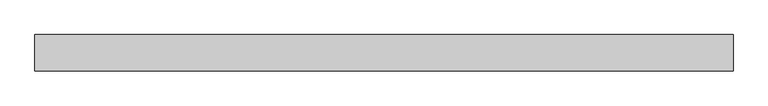
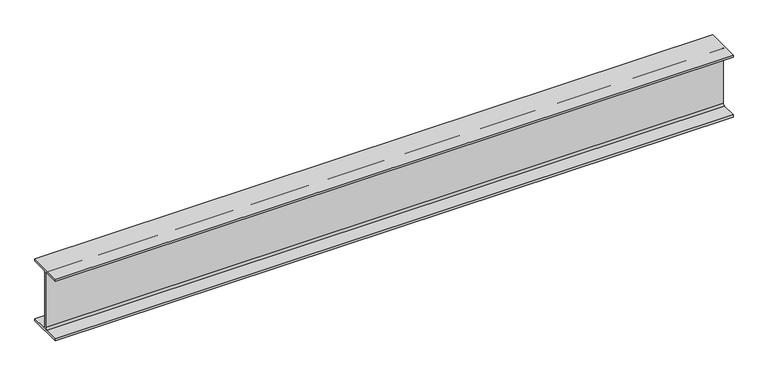
"""IFC4 building model written with IfcOpenShell, lengths in millimetres: beam geometry, Old_Steel Beam_H-KSD3502 : H_SB_ASB_H-250×125x6x9."""

from ifc_helpers import new_model, si_unit, point, frame, frame_2d, origin, place, context, project, spatial, polyline, circle_curve, trimmed, segment, composite_curve, outline, extrude, source, transform, mapped, element, save


def beam_c4c65e90(model_context):
    return source(origin(), model_context, "Body", "SweptSolid", [
        extrude(outline(composite_curve([segment(polyline([(82.5, -141.5), (82.5, -151.7), (-82.5, -151.7), (-82.5, -141.5), (-11.9, -141.5)]), True, "CONTINUOUS"), segment(trimmed(circle_curve(frame_2d((-11.9, -132.6)), 8.9), [point((-11.9, -141.5))], [point((-3.0, -132.6))], True, "CARTESIAN"), True, "CONTINUOUS"), segment(polyline([(-3.0, -132.6), (-3.0, 132.6)]), True, "CONTINUOUS"), segment(trimmed(circle_curve(frame_2d((-11.9, 132.6)), 8.9), [point((-3.0, 132.6))], [point((-11.9, 141.5))], True, "CARTESIAN"), True, "CONTINUOUS"), segment(polyline([(-11.9, 141.5), (-82.5, 141.5), (-82.5, 151.7), (82.5, 151.7), (82.5, 141.5), (11.9, 141.5)]), True, "CONTINUOUS"), segment(trimmed(circle_curve(frame_2d((11.9, 132.6)), 8.9), [point((11.9, 141.5))], [point((3.0, 132.6))], True, "CARTESIAN"), True, "CONTINUOUS"), segment(polyline([(3.0, 132.6), (3.0, -132.6)]), True, "CONTINUOUS"), segment(trimmed(circle_curve(frame_2d((11.9, -132.6)), 8.9), [point((3.0, -132.6))], [point((11.9, -141.5))], True, "CARTESIAN"), True, "CONTINUOUS"), segment(polyline([(11.9, -141.5), (82.5, -141.5)]), True, "CONTINUOUS")], self_intersect=False)), frame((-1494.5360727, 0.0, 0.0), z_axis=(1.0, 0.0, 0.0), x_axis=(0.0, 1.0, 0.0)), (0.0, 0.0, 1.0), 3149.3360727),
    ])


if __name__ == "__main__":
    model = new_model("IFC4")
    model_context = context("Model", 3, world=origin())
    ifc_project = project(units=[si_unit("LENGTHUNIT", "METRE", prefix="MILLI")], contexts=[model_context])
    site = spatial("IfcSite", under=ifc_project)
    building = spatial("IfcBuilding", under=site)
    placement = place(None, origin())
    beam_shape = beam_c4c65e90(model_context)
    element("IfcBeam", 1, ObjectType="Old_Steel Beam_H-KSD3502 : H_SB_ASB_H-250×125x6x9", at=placement, inside=building, context=model_context, shape_type="MappedRepresentation", body=[
        mapped(beam_shape, transform((0.0, 0.0, 0.0), x_axis=(1.0, 0.0, 0.0), y_axis=(0.0, 1.0, 0.0), z_axis=(0.0, 0.0, 1.0))),
    ])
    save(model, "model.ifc")

# Revit data of these elements
# Type "Old_Steel Beam_H-KSD3502 : H_SB_ASB_H-250×125x6x9"
#   Width = 12.5 cm
#   Web Thickness = 0.6 cm
#   Web Fillet = 1.2 cm
#   Warping Constant = 42539.8 cm⁶
#   Torsional Moment of Inertia = 7.8102 cm⁴
#   Torsional Modulus = 1.0 cm³
#   Section Area = 37.66 cm²
#   Plastic Modulus weak axis = 73.1 cm³
#   Plastic Modulus strong axis = 366.0 cm³
#   Perimeter = 0.97 m²/m
#   Nominal Weight = 29.60 kgf/m
#   Moment of Inertia weak axis = 294.00 cm⁴
#   Moment of Inertia strong axis = 4050.00 cm⁴
#   Height = 25.0 cm
#   Flange Thickness = 0.9 cm
#   Elastic Modulus weak axis = 47.0 cm³
#   Elastic Modulus strong axis = 324.0 cm³
#   Centroid Vertical = 12.5 cm
#   Centroid Horizontal = 6.25 cm
#   Length [instance default] = 1.5240 m
#   Structural Material [instance default] = Steel, 45-345
#   Assembly Code = ""
# Element 1 (IfcBeam, "Old_Steel Beam_H-KSD3502 : H_SB_ASB_H-250×125x6x9")
#   Structural Material = none
# Materials
#   "Steel, 45-345": class "Metal", colour RGB 189 187 185, transparency 0, Description = "Steel 345 MPa", Cost = 0
